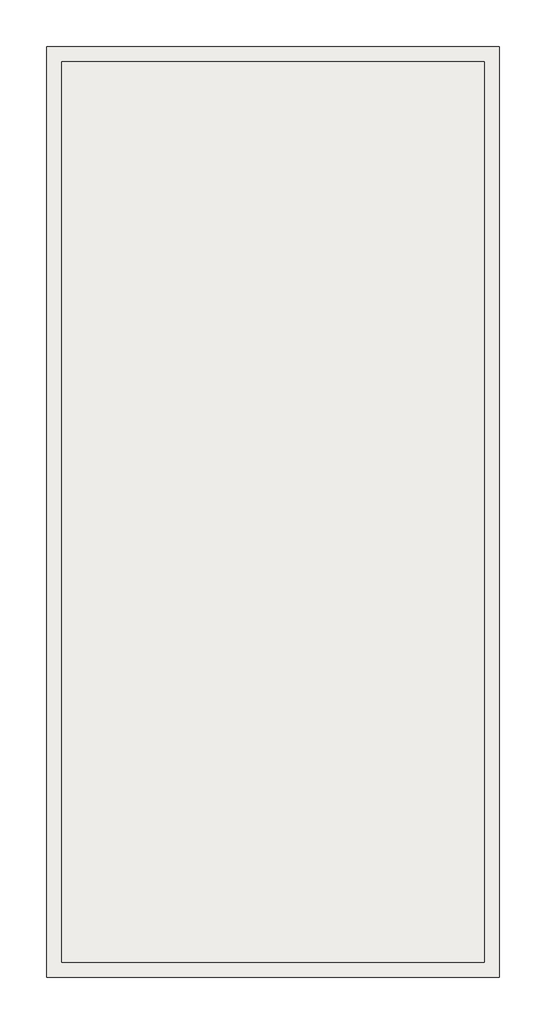
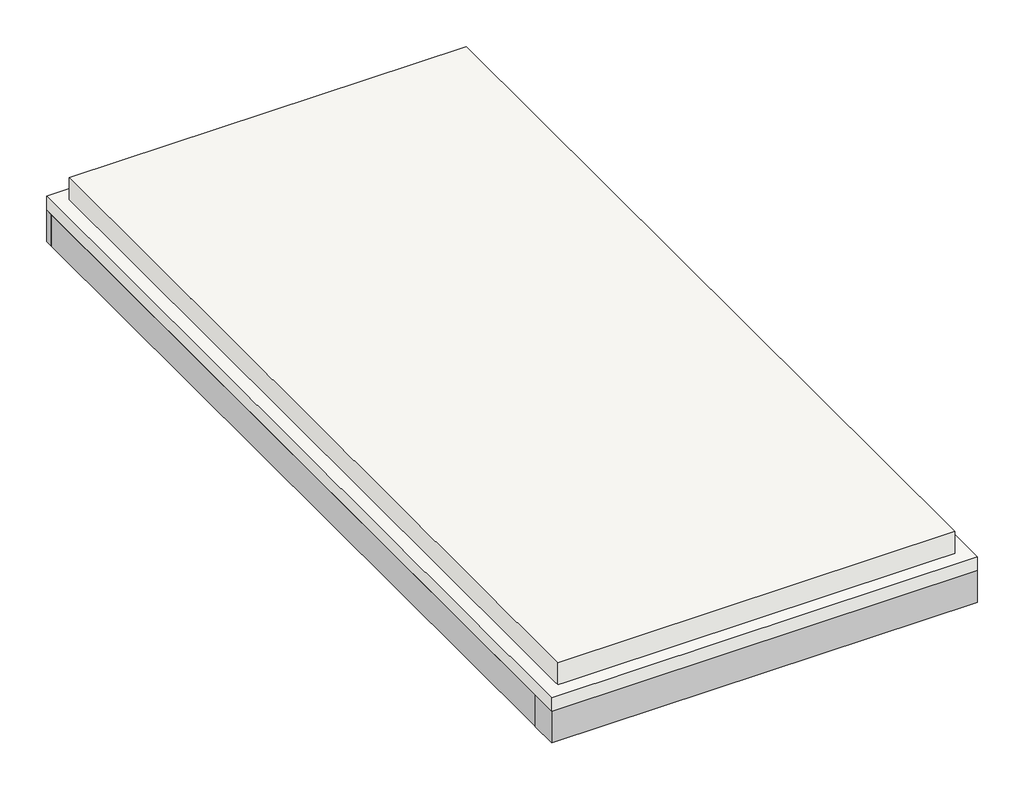
# One storey: 4 beams, 2 slabs.
"""IFC4 building model written with IfcOpenShell, lengths in millimetres."""

from ifc_helpers import new_model, si_unit, frame, origin, place, context, project, spatial, polyline, outline, extrude, faceted_brep, element, save

model = new_model("IFC4")

# Units and contexts
model_context = context("Model", 3, world=origin())
ifc_project = project(units=[si_unit("LENGTHUNIT", "METRE", prefix="MILLI")], contexts=[model_context])

# Site, building, storey
site = spatial("IfcSite", under=ifc_project)
building = spatial("IfcBuilding", under=site)
storey = spatial("IfcBuildingStorey", under=building, Name="P.H ROOF PLAN", Elevation=25100.005241)

# Beams
placement = place(None, origin())
element("IfcBeam", 1, ObjectType="Concrete-Rectangular-Beam : BMS111_RC BEAM_AG_300x500_PRG1", at=placement, inside=storey, context=model_context, shape_type="Brep", body=[
    faceted_brep([(4100.0, 29549.5208589, 24950.005241), (4100.0, 29849.5208589, 24950.005241), (-350.0, 29849.5208589, 24950.005241), (-350.0, 29762.2208589, 24950.005241), (-50.0, 29762.2208589, 24950.005241), (-50.0, 29549.5208589, 24950.005241), (3800.0, 29549.5208589, 24950.005241), (4100.0, 29549.5208589, 24599.905241), (4100.0, 29849.5208589, 24599.905241), (-50.0, 29549.5208589, 24599.905241), (3800.0, 29549.5208589, 24599.905241), (-50.0, 29762.2208589, 24599.905241), (-350.0, 29762.2208589, 24599.905241), (-350.0, 29849.5208589, 24599.905241)], [[[0, 1, 2, 3, 4, 5, 6]], [[1, 0, 7, 8]], [[7, 0, 6, 5, 9, 10]], [[8, 7, 10, 9, 11, 12, 13]], [[1, 8, 13, 2]], [[4, 11, 9, 5]], [[2, 13, 12, 3]], [[11, 4, 3, 12]]]),
])
element("IfcBeam", 2, ObjectType="Concrete-Rectangular-Beam : BMS111_RC BEAM_AG_300x500_PRG1", at=placement, inside=storey, context=model_context, shape_type="Brep", body=[
    faceted_brep([(-351.0, 20999.5208589, 24599.905241), (-351.0, 20699.5208589, 24599.905241), (-351.0, 20699.5208589, 24950.005241), (-351.0, 20999.5208589, 24950.005241), (4100.0, 20699.5208589, 24599.905241), (4100.0, 20999.5208589, 24599.905241), (4100.0, 20999.5208589, 24950.005241), (4100.0, 20699.5208589, 24950.005241), (3800.0, 20999.5208589, 24950.005241), (-50.0, 20999.5208589, 24950.005241), (-350.0, 20999.5208589, 24950.005241), (-350.0, 20999.5208589, 24599.905241), (-50.0, 20999.5208589, 24599.905241), (3800.0, 20999.5208589, 24599.905241)], [[[0, 1, 2, 3]], [[4, 5, 6, 7]], [[3, 2, 7, 6, 8, 9, 10]], [[1, 4, 7, 2]], [[1, 0, 11, 12, 13, 5, 4]], [[5, 13, 12, 11, 0, 3, 10, 9, 8, 6]]]),
])
element("IfcBeam", 3, ObjectType="Concrete-Rectangular-Beam : BMS111_RC BEAM_AG_300x500_PRG1", at=placement, inside=storey, context=model_context, shape_type="Brep", body=[
    faceted_brep([(3800.0, 20999.5208589, 24950.005241), (4100.0, 20999.5208589, 24950.005241), (4100.0, 29549.5208589, 24950.005241), (3800.0, 29549.5208589, 24950.005241), (3800.0, 27099.5208589, 24950.005241), (3800.0, 26799.5208589, 24950.005241), (3800.0, 20999.5208589, 24599.905241), (4100.0, 20999.5208589, 24599.905241), (3800.0, 29549.5208589, 24599.905241), (4100.0, 29549.5208589, 24599.905241)], [[[0, 1, 2, 3, 4, 5]], [[1, 0, 6, 7]], [[6, 0, 5, 4, 3, 8]], [[7, 6, 8, 9]], [[1, 7, 9, 2]], [[3, 2, 9, 8]]]),
])
element("IfcBeam", 4, ObjectType="Concrete-Rectangular-Beam : BMS111_RC BEAM_AG_300x500_PRG1", at=placement, inside=storey, context=model_context, shape_type="Brep", body=[
    faceted_brep([(-350.0, 20999.5208589, 24950.005241), (-50.0, 20999.5208589, 24950.005241), (-50.0, 26799.5208589, 24950.005241), (-50.0, 27099.5208589, 24950.005241), (-50.0, 29549.5208589, 24950.005241), (-50.0, 29762.2208589, 24950.005241), (-350.0, 29762.2208589, 24950.005241), (-350.0, 20999.5208589, 24599.905241), (-50.0, 20999.5208589, 24599.905241), (-50.0, 29762.2208589, 24599.905241), (-350.0, 29762.2208589, 24599.905241), (-50.0, 29549.5208589, 24599.905241)], [[[0, 1, 2, 3, 4, 5, 6]], [[7, 8, 1, 0]], [[9, 10, 6, 5]], [[10, 7, 0, 6]], [[10, 9, 11, 8, 7]], [[8, 11, 9, 5, 4, 3, 2, 1]]]),
])

# Slabs
element("IfcSlab", 5, ObjectType="SLS111_RC Floor_T150 - PRS1", at=placement, inside=storey, context=model_context, shape_type="Brep", body=[
    faceted_brep([(4101.0, 29849.5208589, 24950.005241), (4101.0, 20698.5208589, 24950.005241), (-351.0, 20698.5208589, 24950.005241), (-351.0, 20699.5208589, 24950.005241), (-351.0, 20999.5208589, 24950.005241), (-351.0, 29849.5208589, 24950.005241), (-350.0, 29849.5208589, 24950.005241), (4100.0, 29849.5208589, 24950.005241), (4101.0, 29849.5208589, 25100.005241), (-351.0, 29849.5208589, 25100.005241), (-351.0, 20698.5208589, 25100.005241), (4101.0, 20698.5208589, 25100.005241), (4101.0, 20849.5208589, 25100.005241)], [[[0, 1, 2, 3, 4, 5, 6, 7]], [[8, 9, 10, 11, 12]], [[1, 0, 8, 12, 11]], [[2, 1, 11, 10]], [[5, 4, 3, 2, 10, 9]], [[0, 7, 6, 5, 9, 8]]]),
])
element("IfcSlab", 6, ObjectType="SLFC181_WF_Insulation_Protection_T60", at=placement, inside=storey, context=model_context, shape_type="SweptSolid", body=[
    extrude(outline(polyline([(3950.0, 29699.5208589), (3950.0, 20849.5208589), (-201.0, 20849.5208589), (-201.0, 29699.5208589), (3950.0, 29699.5208589)])), frame((0.0, 0.0, 25100.005241), z_axis=(0.0, 0.0, 1.0), x_axis=(1.0, 0.0, 0.0)), (0.0, 0.0, 1.0), 242.0),
])

save(model, "model.ifc")

# Revit data of these elements
# Type "Concrete-Rectangular-Beam : BMS111_RC BEAM_AG_300x500_PRG1"
#   Type Mark = "PRG1"
#   중앙부 하부근 = "2-D20"
#   중앙부 상부근 = "2-D20"
#   중앙부 보조근 = ""
#   중앙부 늑근 = "2-D10 @200"
#   외단부 하부근 = "2-D20"
#   외단부 상부근 = "2-D20"
#   외단부 보조근 = ""
#   외단부 늑근 = "2-D10 @100"
#   부호 = "PRG1"
#   내단부 하부근 = "2-D20"
#   내단부 상부근 = "2-D20"
#   내단부 보조근 = ""
#   내단부 늑근 = "2-D10 @100"
#   ALL 하부근 = ""
#   ALL 상부근 = ""
#   ALL 보조근 = ""
#   ALL 늑근 = ""
#   Width = 300 mm
#   Height = 500 mm
#   Length [instance default] = 1524 mm
#   b = 300 mm
#   h = 500 mm
#   Structural Material [instance default] = 콘크리트 - 현장타설 콘크리트
#   hec_material3 [instance default] = none
#   hec_material2 [instance default] = none
#   hec_material1 [instance default] = none
#   Assembly Code = ""
# Type "SLS111_RC Floor_T150 - PRS1"
#   Keynote = ""
#   Type Comments = "구조_콘크리트"
#   Type Mark = "PRS1"
#   Function = 0
#   Layers, outside or top first: 150 mm "A03AD032-00007_Structural Concrete_25MPa-30MPa" (function 1)
# Type "SLFC181_WF_Insulation_Protection_T60"
#   Assembly Code = "1S1"
#   Function = 0
#   Layers, outside or top first: 60 mm "A04AP089-00001_Protective Concrete w/ Steel Trowel Finish" (function 1); 0 mm "A04AP038-00002_Welded Wire Fabric" (function 100); 1 mm "A04AP012-00001_PE Sheet (Vapor Barrier)_Roof" (function 4); 180 mm "A04AP088-00001_Roof_Rigid Extruded Polystyrene Foam Insulation" (function 3); 1 mm "A04AP000-00001_Roof_Waterproofing Membrane" (function 4)
# Elements 1, 2, 3, 4 (IfcBeam, "Concrete-Rectangular-Beam : BMS111_RC BEAM_AG_300x500_PRG1")
#   Comments = ""
#   hec_material3 = none
#   hec_material2 = none
#   hec_material1 = none
#   Structural Material = A03AD032-00007_Structural Concrete_25MPa-30MPa
#   Phase Created = New Construction
#   Materials on its faces: "A03AD032-00007_Structural Concrete_25MPa-30MPa"
# Element 5 (IfcSlab, "SLS111_RC Floor_T150 - PRS1")
#   Comments = ""
#   Height Offset From Level = 0 mm
#   built-in parameter 1001954 = 1
#   Phase Created = New Construction
#   Materials on its faces: "A03AD032-00007_Structural Concrete_25MPa-30MPa"
# Element 6 (IfcSlab, "SLFC181_WF_Insulation_Protection_T60")
#   Height Offset From Level = 242 mm
#   Phase Created = New Construction
#   Materials on its faces: "A04AP000-00001_Roof_Waterproofing Membrane", "A04AP089-00001_Protective Concrete w/ Steel Trowel Finish"
# Materials
#   "콘크리트 - 현장타설 콘크리트": class "콘크리트", colour RGB 192 192 192, transparency 0
#   "A03AD032-00007_Structural Concrete_25MPa-30MPa": class "Concrete", colour RGB 176 176 176, transparency 0, Keynote = "09910.A1", Description = "ACRYLIC EMULSION PAINT ON\nFAIR FACED CONC.", W00) Work Master Code = "A03AD032-00007", W01) Work Master_Lv1 = "Concrete Work", W02) Work Master_Lv2 = "Superstructure Work", W03) Work Master_Spec.1 = "Structural Concrete", W04) Work Master_Spec.2 = "Cement Type-1", W05) Work Master_Spec.3 = "25MPa < F'c (Cylinder Strength) ≤ 30MPa", Cost = 0
#   "A04AP089-00001_Protective Concrete w/ Steel Trowel Finish": class "Concrete", colour RGB 176 176 176, transparency 0, Description = "PROTECTION CONCRETE MIN.60(W/#8-150x150 WIRE MESH)", W00) Work Master Code = "A04AP089-00001", W01) Work Master_Lv1 = "Finishing Work", W02) Work Master_Lv2 = "Roof Work", W03) Work Master_Spec.1 = "Protective Concrete w/ Steel Trowel Finish", Cost = 0
#   "A04AP038-00002_Welded Wire Fabric": class "Concrete", colour RGB 176 176 176, transparency 0, Description = "Welded Wire Fabric", W00) Work Master Code = "A04AP038-00002", W01) Work Master_Lv1 = "Finishing Work", W02) Work Master_Lv2 = "Roof Work", W03) Work Master_Spec.1 = "Welded Wire Fabric", W04) Work Master_Spec.2 = "DIA>6mm", Cost = 0
#   "A04AP012-00001_PE Sheet (Vapor Barrier)_Roof": class "Finish", colour RGB 128 128 64, transparency 0, Description = "THK.0.1 PE SHEET 2PLY", W00) Work Master Code = "A04AP012-00001", W01) Work Master_Lv1 = "Finishing Work", W02) Work Master_Lv2 = "Roof Work", W03) Work Master_Spec.1 = "PE Sheet (Vapor Barrier)", Cost = 0
#   "A04AP088-00001_Roof_Rigid Extruded Polystyrene Foam Insulation": class "Insulation", colour RGB 255 255 217, transparency 0, Description = "THK.180 RIGID EXTRUDED POLYSTYEREN FORM INSULATION", W00) Work Master Code = "A04AP088-00001", W01) Work Master_Lv1 = "Finishing Work", W02) Work Master_Lv2 = "Roof Work", W03) Work Master_Spec.1 = "Roof Insulation", W04) Work Master_Spec.2 = "Rigid Extruded Polystyrene Foam Insulation", W05) Work Master_Spec.3 = "50mm≤THK<75mm", Cost = 0
#   "A04AP000-00001_Roof_Waterproofing Membrane": class "Plastic", colour RGB 127 127 127, transparency 0, Description = "WATERPROOFING MEMBRANE", W00) Work Master Code = "A04AP000-00001", W01) Work Master_Lv1 = "Finishing Work", W02) Work Master_Lv2 = "Roof Work", W03) Work Master_Spec.1 = "Waterproofing Membrane", W04) Work Master_Spec.2 = "EPDM(or Equivalent)", W05) Work Master_Spec.3 = "w/ Accessories", Cost = 0
